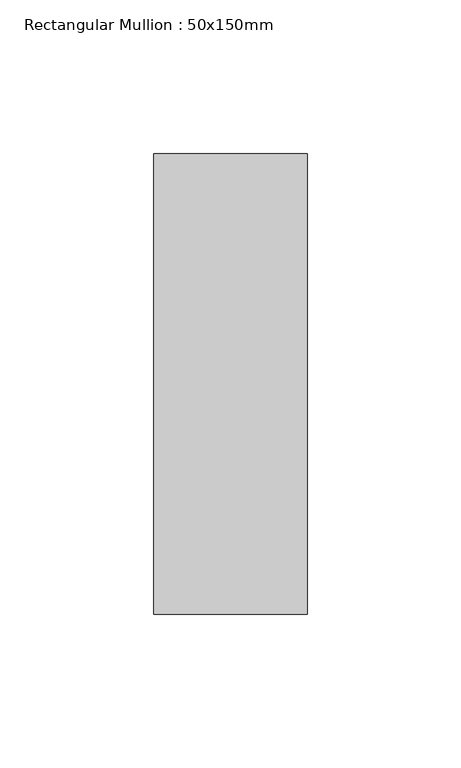
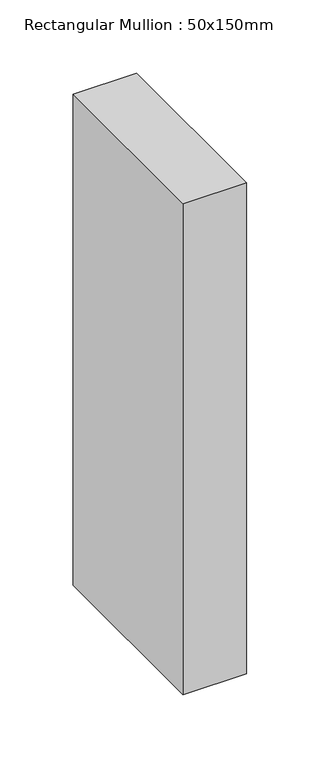
"""IFC4 building model written with IfcOpenShell, lengths in millimetres: member geometry, Rectangular Mullion : 50x150mm."""

from ifc_helpers import new_model, si_unit, frame, origin, place, context, project, spatial, polyline, outline, extrude, source, transform, mapped, element, save


def rectangular_mullion_50x150mm_c82d2d4e(model_context):
    return source(origin(), model_context, "Body", "SweptSolid", [
        extrude(outline(polyline([(0.0, 75.0), (0.0, -75.0), (-50.0, -75.0), (-50.0, 75.0), (0.0, 75.0)])), frame((0.0, 0.0, -408.4078826), z_axis=(0.0, 0.0, 1.0), x_axis=(1.0, 0.0, 0.0)), (0.0, 0.0, 1.0), 408.4078826),
    ])


if __name__ == "__main__":
    model = new_model("IFC4")
    model_context = context("Model", 3, world=origin())
    ifc_project = project(units=[si_unit("LENGTHUNIT", "METRE", prefix="MILLI")], contexts=[model_context])
    site = spatial("IfcSite", under=ifc_project)
    building = spatial("IfcBuilding", under=site)
    placement = place(None, origin())
    rectangular_mullion_50x150mm_shape = rectangular_mullion_50x150mm_c82d2d4e(model_context)
    element("IfcMember", 1, ObjectType="Rectangular Mullion : 50x150mm", at=placement, inside=building, context=model_context, shape_type="MappedRepresentation", body=[
        mapped(rectangular_mullion_50x150mm_shape, transform((0.0, 0.0, 0.0), x_axis=(1.0, 0.0, 0.0), y_axis=(0.0, 1.0, 0.0), z_axis=(0.0, 0.0, 1.0))),
    ])
    save(model, "model.ifc")

# Revit data of these elements
# Type "Rectangular Mullion : 50x150mm"
#   Keynote = "H11"
#   built-in parameter 1007304 = 0.492126 (stored number, unit not read)
#   built-in parameter 1007301 = 0.082021 (stored number, unit not read)
#   built-in parameter 1007300 = 0.082021 (stored number, unit not read)
# Element 1 (IfcMember, "Rectangular Mullion : 50x150mm")
#   Materials on its faces: "Aluminium"
# Materials
#   "Aluminium": class "Metal", colour RGB 247 247 247, transparency 0, Description = "Aluminium 6061", Cost = 0
